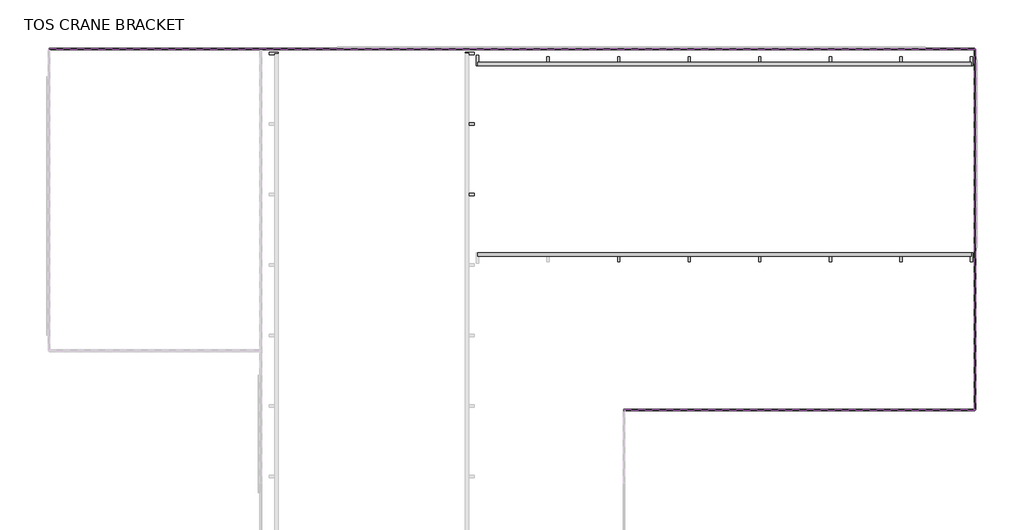
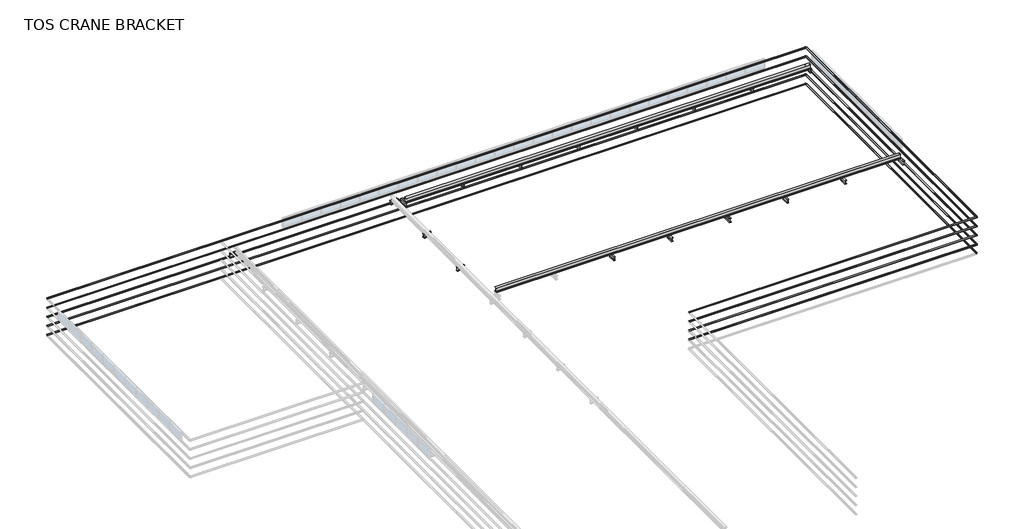
# One storey, part 3 of 3: 34 beams.
"""IFC4 building model written with IfcOpenShell, lengths in millimetres."""

import ifcopenshell
import ifcopenshell.guid

model = None  # the IFC model being written
_history = None  # IfcOwnerHistory: only IFC2X3 demands one
_inside = {}  # id of a spatial element -> (the spatial element, [elements in it])
_under = {}  # id of a project, library or spatial element -> (it, [spatial elements below it])
_declared = {}  # id of a project -> (the project, [libraries it declares])
_typed = {}  # id of a type object -> (the type object, [elements of that type])
_made_of = {}  # id of a material, layer set ... -> (it, [elements and type objects made of it])


def new_model(schema):
    """Start an empty IFC model of exactly this schema.

    Asked for "IFC4X3", IfcOpenShell would pick the latest addendum, in which some entities
    have other attributes; the version numbers below select the first issue.
    IFC2X3 requires an IfcOwnerHistory on every rooted entity: one is made here for all.
    """
    global model, _history
    if schema == "IFC4X3":
        model = ifcopenshell.file(schema_version=(4, 3, 0, 0))
    else:
        model = ifcopenshell.file(schema=schema)
    _inside.clear()
    _under.clear()
    _declared.clear()
    _typed.clear()
    _made_of.clear()
    _history = None
    if model.schema == "IFC2X3":
        org = make("IfcOrganization", Name="unknown")
        user = make(
            "IfcPersonAndOrganization",
            ThePerson=make("IfcPerson", FamilyName="unknown"),
            TheOrganization=org,
        )
        app = make(
            "IfcApplication",
            ApplicationDeveloper=org,
            Version="unknown",
            ApplicationFullName="unknown",
            ApplicationIdentifier="unknown",
        )
        _history = make(
            "IfcOwnerHistory",
            OwningUser=user,
            OwningApplication=app,
            ChangeAction="ADDED",
            CreationDate=0,
        )
    return model


def make(cls, **values):
    """One entity of the class cls with the attributes given. An attribute that is None is left unset."""
    return model.create_entity(
        cls, **{name: value for name, value in values.items() if value is not None}
    )


def rooted(cls, **values):
    """An entity with a GlobalId (a new one), such as an element, a storey or a relation."""
    return make(cls, GlobalId=ifcopenshell.guid.new(), OwnerHistory=_history, **values)


def si_unit(unit_type, name, prefix=None):
    """IfcSIUnit, for example si_unit("LENGTHUNIT", "METRE", prefix="MILLI")."""
    return make("IfcSIUnit", UnitType=unit_type, Prefix=prefix, Name=name)


def assignment(units):
    """IfcUnitAssignment: the units of a project."""
    return None if units is None else make("IfcUnitAssignment", Units=units)


def point(xyz):
    """IfcCartesianPoint."""
    return None if xyz is None else make("IfcCartesianPoint", Coordinates=xyz)


def direction(xyz):
    """IfcDirection."""
    return None if xyz is None else make("IfcDirection", DirectionRatios=xyz)


def frame(location, z_axis=None, x_axis=None):
    """IfcAxis2Placement3D, a coordinate frame: its origin and axes. An axis left out is left unset."""
    return make(
        "IfcAxis2Placement3D",
        Location=point(location),
        Axis=direction(z_axis),
        RefDirection=direction(x_axis),
    )


def frame_2d(location, x_axis=None):
    """IfcAxis2Placement2D, a coordinate frame in the plane: its origin and x axis."""
    return make(
        "IfcAxis2Placement2D", Location=point(location), RefDirection=direction(x_axis)
    )


def origin():
    """The frame at (0, 0, 0) with its axes left unset."""
    return frame((0.0, 0.0, 0.0))


def place(relative_to, where):
    """IfcLocalPlacement: puts the frame where relative to a parent placement (None: the world)."""
    return make(
        "IfcLocalPlacement", PlacementRelTo=relative_to, RelativePlacement=where
    )


def context(
    kind, dimensions, precision=None, world=None, true_north=None, identifier=None
):
    """IfcGeometricRepresentationContext, for example the 3D "Model" context."""
    return make(
        "IfcGeometricRepresentationContext",
        ContextIdentifier=identifier,
        ContextType=kind,
        CoordinateSpaceDimension=dimensions,
        Precision=precision,
        WorldCoordinateSystem=world,
        TrueNorth=true_north,
    )


def project(units=None, contexts=None):
    """IfcProject with its units and contexts."""
    return rooted(
        "IfcProject",
        Name="project",
        RepresentationContexts=contexts,
        UnitsInContext=assignment(units),
    )


def spatial(cls, under=None, at=None, **own):
    """A site, building, storey or space (cls), placed at a placement, below another one or the project."""
    s = rooted(cls, ObjectPlacement=at, **own)
    if under is not None:
        _under.setdefault(under.id(), (under, []))[1].append(s)
    return s


def polyline(points):
    """IfcPolyline through the points."""
    return make("IfcPolyline", Points=[point(p) for p in points])


def circle_curve(where, radius):
    """IfcCircle in the frame where."""
    return make("IfcCircle", Position=where, Radius=radius)


def trimmed(basis, trim1, trim2, sense, master):
    """IfcTrimmedCurve: the piece of a basis curve between two trims."""
    return make(
        "IfcTrimmedCurve",
        BasisCurve=basis,
        Trim1=trim1,
        Trim2=trim2,
        SenseAgreement=sense,
        MasterRepresentation=master,
    )


def segment(curve, same_sense, transition):
    """IfcCompositeCurveSegment."""
    return make(
        "IfcCompositeCurveSegment",
        Transition=transition,
        SameSense=same_sense,
        ParentCurve=curve,
    )


def composite_curve(segments, self_intersect=None):
    """IfcCompositeCurve: segments joined end to end."""
    return make("IfcCompositeCurve", Segments=segments, SelfIntersect=self_intersect)


def outline(outer, holes=None, kind="AREA"):
    """IfcArbitraryClosedProfileDef: a profile drawn as a closed curve; with holes, ...WithVoids."""
    if holes is None:
        return make("IfcArbitraryClosedProfileDef", ProfileType=kind, OuterCurve=outer)
    return make(
        "IfcArbitraryProfileDefWithVoids",
        ProfileType=kind,
        OuterCurve=outer,
        InnerCurves=holes,
    )


def extrude(swept, where, along, depth):
    """IfcExtrudedAreaSolid: the profile swept, set in the frame where, extruded along a direction by depth."""
    return make(
        "IfcExtrudedAreaSolid",
        SweptArea=swept,
        Position=where,
        ExtrudedDirection=direction(along),
        Depth=depth,
    )


def shape(context_of_items, identifier, shape_type, items):
    """IfcShapeRepresentation: the items that make up one representation, for example the "Body"."""
    return make(
        "IfcShapeRepresentation",
        ContextOfItems=context_of_items,
        RepresentationIdentifier=identifier,
        RepresentationType=shape_type,
        Items=items,
    )


def source(mapping_origin, context_of_items, identifier, shape_type, items):
    """IfcRepresentationMap: a shape defined once, which mapped items show again and again."""
    return make(
        "IfcRepresentationMap",
        MappingOrigin=mapping_origin,
        MappedRepresentation=shape(context_of_items, identifier, shape_type, items),
    )


def transform(
    local_origin,
    x_axis=None,
    y_axis=None,
    z_axis=None,
    scale=None,
    scale2=None,
    scale3=None,
    uniform=True,
):
    """IfcCartesianTransformationOperator3D, or its non-uniform kind. x_axis, y_axis, z_axis: its Axis1, 2, 3."""
    if uniform:
        return make(
            "IfcCartesianTransformationOperator3D",
            Axis1=direction(x_axis),
            Axis2=direction(y_axis),
            LocalOrigin=point(local_origin),
            Scale=scale,
            Axis3=direction(z_axis),
        )
    return make(
        "IfcCartesianTransformationOperator3DnonUniform",
        Axis1=direction(x_axis),
        Axis2=direction(y_axis),
        LocalOrigin=point(local_origin),
        Scale=scale,
        Axis3=direction(z_axis),
        Scale2=scale2,
        Scale3=scale3,
    )


def mapped(mapping_source, mapping_target):
    """IfcMappedItem: shows the shape of a source again, moved by a transform."""
    return make(
        "IfcMappedItem", MappingSource=mapping_source, MappingTarget=mapping_target
    )


def made_of(thing, what):
    """Note that an element or type object is made of a material, layer set ...; save() writes the relation."""
    if what is not None:
        _made_of.setdefault(what.id(), (what, []))[1].append(thing)
    return thing


def element(
    cls,
    number,
    at=None,
    inside=None,
    cuts=None,
    type_object=None,
    material=None,
    context=None,
    identifier="Body",
    shape_type=None,
    held_by="IfcProductDefinitionShape",
    body=None,
    shapes=None,
    **own,
):
    """One element of the class cls, such as IfcWall. Its Tag is "e" and its number.

    at: its placement. inside: the storey or other place that contains it. cuts: it is an
    opening in that element (IfcRelVoidsElement). A single representation is given by context,
    identifier, shape_type and body (its items); several are given by shapes. held_by: the class
    of the entity that holds the representations. save() writes the other relations.
    """
    e = rooted(cls, Tag="e%d" % number, ObjectPlacement=at, **own)
    if body is not None:
        shapes = [shape(context, identifier, shape_type, body)]
    if shapes is not None:
        e.Representation = make(held_by, Representations=shapes)
    if inside is not None:
        _inside.setdefault(inside.id(), (inside, []))[1].append(e)
    if cuts is not None:
        rooted(
            "IfcRelVoidsElement", RelatingBuildingElement=cuts, RelatedOpeningElement=e
        )
    if type_object is not None:
        _typed.setdefault(type_object.id(), (type_object, []))[1].append(e)
    return made_of(e, material)


def aggregate(whole, parts):
    """IfcRelAggregates: a whole, such as a stair, and the parts it consists of."""
    return rooted("IfcRelAggregates", RelatingObject=whole, RelatedObjects=parts)


def save(model, path):
    """Write the relations noted so far, then the file.

    IfcRelAggregates (storeys below a building ...), IfcRelContainedInSpatialStructure (elements
    in a storey), IfcRelDefinesByType, IfcRelAssociatesMaterial and IfcRelDeclares: one each for
    every whole, place, type object, material and project.
    """
    for whole, parts in _under.values():
        aggregate(whole, parts)
    for where, things in _inside.values():
        rooted(
            "IfcRelContainedInSpatialStructure",
            RelatedElements=things,
            RelatingStructure=where,
        )
    for kind, things in _typed.values():
        rooted("IfcRelDefinesByType", RelatedObjects=things, RelatingType=kind)
    for what, things in _made_of.values():
        rooted("IfcRelAssociatesMaterial", RelatedObjects=things, RelatingMaterial=what)
    for by, libraries in _declared.values():
        rooted("IfcRelDeclares", RelatingContext=by, RelatedDefinitions=libraries)
    model.write(path)


def beam_a081c7c9(model_context):
    return source(origin(), model_context, "Body", "SweptSolid", [
        extrude(outline(composite_curve([segment(polyline([(100.0, -187.0), (100.0, -200.0), (-100.0, -200.0), (-100.0, -187.0), (-20.0, -187.0)]), True, "CONTINUOUS"), segment(trimmed(circle_curve(frame_2d((-20.0, -171.0)), 16.0), [point((-20.0, -187.0))], [point((-4.0, -171.0))], True, "CARTESIAN"), True, "CONTINUOUS"), segment(polyline([(-4.0, -171.0), (-4.0, 171.0)]), True, "CONTINUOUS"), segment(trimmed(circle_curve(frame_2d((-20.0, 171.0)), 16.0), [point((-4.0, 171.0))], [point((-20.0, 187.0))], True, "CARTESIAN"), True, "CONTINUOUS"), segment(polyline([(-20.0, 187.0), (-100.0, 187.0), (-100.0, 200.0), (100.0, 200.0), (100.0, 187.0), (20.0, 187.0)]), True, "CONTINUOUS"), segment(trimmed(circle_curve(frame_2d((20.0, 171.0)), 16.0), [point((20.0, 187.0))], [point((4.0, 171.0))], True, "CARTESIAN"), True, "CONTINUOUS"), segment(polyline([(4.0, 171.0), (4.0, -171.0)]), True, "CONTINUOUS"), segment(trimmed(circle_curve(frame_2d((20.0, -171.0)), 16.0), [point((4.0, -171.0))], [point((20.0, -187.0))], True, "CARTESIAN"), True, "CONTINUOUS"), segment(polyline([(20.0, -187.0), (100.0, -187.0)]), True, "CONTINUOUS")], self_intersect=False)), frame((-236.0, 0.0, 0.0), z_axis=(1.0, 0.0, 0.0), x_axis=(0.0, 1.0, 0.0)), (0.0, 0.0, 1.0), 766.0),
    ])


def beam_d36fe593(model_context):
    return source(origin(), model_context, "Body", "SweptSolid", [
        extrude(outline(composite_curve([segment(polyline([(-100.0, -187.0), (-20.0, -187.0)]), True, "CONTINUOUS"), segment(trimmed(circle_curve(frame_2d((-20.0, -171.0)), 16.0), [point((-20.0, -187.0))], [point((-4.0, -171.0))], True, "CARTESIAN"), True, "CONTINUOUS"), segment(polyline([(-4.0, -171.0), (-4.0, 171.0)]), True, "CONTINUOUS"), segment(trimmed(circle_curve(frame_2d((-20.0, 171.0)), 16.0), [point((-4.0, 171.0))], [point((-20.0, 187.0))], True, "CARTESIAN"), True, "CONTINUOUS"), segment(polyline([(-20.0, 187.0), (-100.0, 187.0), (-100.0, 200.0), (100.0, 200.0), (100.0, 187.0), (20.0, 187.0)]), True, "CONTINUOUS"), segment(trimmed(circle_curve(frame_2d((20.0, 171.0)), 16.0), [point((20.0, 187.0))], [point((4.0, 171.0))], True, "CARTESIAN"), True, "CONTINUOUS"), segment(polyline([(4.0, 171.0), (4.0, -171.0)]), True, "CONTINUOUS"), segment(trimmed(circle_curve(frame_2d((20.0, -171.0)), 16.0), [point((4.0, -171.0))], [point((20.0, -187.0))], True, "CARTESIAN"), True, "CONTINUOUS"), segment(polyline([(20.0, -187.0), (100.0, -187.0), (100.0, -200.0), (-100.0, -200.0), (-100.0, -187.0)]), True, "CONTINUOUS")], self_intersect=False)), frame((-236.0, 0.0, 0.0), z_axis=(1.0, 0.0, 0.0), x_axis=(0.0, 1.0, 0.0)), (0.0, 0.0, 1.0), 766.0),
    ])


def beam_cf9155bb(model_context):
    return source(origin(), model_context, "Body", "SweptSolid", [
        extrude(outline(composite_curve([segment(polyline([(100.0, -187.0), (100.0, -200.0), (-100.0, -200.0), (-100.0, -187.0), (-20.0, -187.0)]), True, "CONTINUOUS"), segment(trimmed(circle_curve(frame_2d((-20.0, -171.0)), 16.0), [point((-20.0, -187.0))], [point((-4.0, -171.0))], True, "CARTESIAN"), True, "CONTINUOUS"), segment(polyline([(-4.0, -171.0), (-4.0, 171.0)]), True, "CONTINUOUS"), segment(trimmed(circle_curve(frame_2d((-20.0, 171.0)), 16.0), [point((-4.0, 171.0))], [point((-20.0, 187.0))], True, "CARTESIAN"), True, "CONTINUOUS"), segment(polyline([(-20.0, 187.0), (-100.0, 187.0), (-100.0, 200.0), (100.0, 200.0), (100.0, 187.0), (20.0, 187.0)]), True, "CONTINUOUS"), segment(trimmed(circle_curve(frame_2d((20.0, 171.0)), 16.0), [point((20.0, 187.0))], [point((4.0, 171.0))], True, "CARTESIAN"), True, "CONTINUOUS"), segment(polyline([(4.0, 171.0), (4.0, -171.0)]), True, "CONTINUOUS"), segment(trimmed(circle_curve(frame_2d((20.0, -171.0)), 16.0), [point((4.0, -171.0))], [point((20.0, -187.0))], True, "CARTESIAN"), True, "CONTINUOUS"), segment(polyline([(20.0, -187.0), (100.0, -187.0)]), True, "CONTINUOUS")], self_intersect=False)), frame((-380.0, 0.0, 0.0), z_axis=(1.0, 0.0, 0.0), x_axis=(0.0, 1.0, 0.0)), (0.0, 0.0, 1.0), 910.0),
    ])


def beam_632170ba(model_context):
    return source(origin(), model_context, "Body", "SweptSolid", [
        extrude(outline(composite_curve([segment(polyline([(150.0, -226.0), (150.0, -244.0), (-150.0, -244.0), (-150.0, -226.0), (-31.5, -226.0)]), True, "CONTINUOUS"), segment(trimmed(circle_curve(frame_2d((-31.5, -200.0)), 26.0), [point((-31.5, -226.0))], [point((-5.5, -200.0))], True, "CARTESIAN"), True, "CONTINUOUS"), segment(polyline([(-5.5, -200.0), (-5.5, 200.0)]), True, "CONTINUOUS"), segment(trimmed(circle_curve(frame_2d((-31.5, 200.0)), 26.0), [point((-5.5, 200.0))], [point((-31.5, 226.0))], True, "CARTESIAN"), True, "CONTINUOUS"), segment(polyline([(-31.5, 226.0), (-150.0, 226.0), (-150.0, 244.0), (150.0, 244.0), (150.0, 226.0), (31.5, 226.0)]), True, "CONTINUOUS"), segment(trimmed(circle_curve(frame_2d((31.5, 200.0)), 26.0), [point((31.5, 226.0))], [point((5.5, 200.0))], True, "CARTESIAN"), True, "CONTINUOUS"), segment(polyline([(5.5, 200.0), (5.5, -200.0)]), True, "CONTINUOUS"), segment(trimmed(circle_curve(frame_2d((31.5, -200.0)), 26.0), [point((5.5, -200.0))], [point((31.5, -226.0))], True, "CARTESIAN"), True, "CONTINUOUS"), segment(polyline([(31.5, -226.0), (150.0, -226.0)]), True, "CONTINUOUS")], self_intersect=False)), frame((-20987.2, 0.0, 0.0), z_axis=(1.0, 0.0, 0.0), x_axis=(0.0, 1.0, 0.0)), (0.0, 0.0, 1.0), 41974.4),
    ])


def beam_85a0d6c7(model_context):
    return source(origin(), model_context, "Body", "SweptSolid", [
        extrude(outline(composite_curve([segment(polyline([(-150.0, -226.0), (-31.5, -226.0)]), True, "CONTINUOUS"), segment(trimmed(circle_curve(frame_2d((-31.5, -200.0)), 26.0), [point((-31.5, -226.0))], [point((-5.5, -200.0))], True, "CARTESIAN"), True, "CONTINUOUS"), segment(polyline([(-5.5, -200.0), (-5.5, 200.0)]), True, "CONTINUOUS"), segment(trimmed(circle_curve(frame_2d((-31.5, 200.0)), 26.0), [point((-5.5, 200.0))], [point((-31.5, 226.0))], True, "CARTESIAN"), True, "CONTINUOUS"), segment(polyline([(-31.5, 226.0), (-150.0, 226.0), (-150.0, 244.0), (150.0, 244.0), (150.0, 226.0), (31.5, 226.0)]), True, "CONTINUOUS"), segment(trimmed(circle_curve(frame_2d((31.5, 200.0)), 26.0), [point((31.5, 226.0))], [point((5.5, 200.0))], True, "CARTESIAN"), True, "CONTINUOUS"), segment(polyline([(5.5, 200.0), (5.5, -200.0)]), True, "CONTINUOUS"), segment(trimmed(circle_curve(frame_2d((31.5, -200.0)), 26.0), [point((5.5, -200.0))], [point((31.5, -226.0))], True, "CARTESIAN"), True, "CONTINUOUS"), segment(polyline([(31.5, -226.0), (150.0, -226.0), (150.0, -244.0), (-150.0, -244.0), (-150.0, -226.0)]), True, "CONTINUOUS")], self_intersect=False)), frame((-20987.2, 0.0, 0.0), z_axis=(1.0, 0.0, 0.0), x_axis=(0.0, 1.0, 0.0)), (0.0, 0.0, 1.0), 41974.4),
    ])


def steel_framing_lc_01a803ec(model_context):
    return source(origin(), model_context, "Body", "SweptSolid", [
        extrude(outline(composite_curve([segment(polyline([(18.6, 67.0), (18.6, -67.0)]), True, "CONTINUOUS"), segment(trimmed(circle_curve(frame_2d((10.6, -67.0)), 8.0), [point((18.6, -67.0))], [point((10.6, -75.0))], False, "CARTESIAN"), True, "CONTINUOUS"), segment(polyline([(10.6, -75.0), (-48.4, -75.0)]), True, "CONTINUOUS"), segment(trimmed(circle_curve(frame_2d((-48.4, -67.0)), 8.0), [point((-48.4, -75.0))], [point((-56.4, -67.0))], False, "CARTESIAN"), True, "CONTINUOUS"), segment(polyline([(-56.4, -67.0), (-56.4, -50.0), (-53.2, -50.0), (-53.2, -67.0)]), True, "CONTINUOUS"), segment(trimmed(circle_curve(frame_2d((-48.4, -67.0)), 4.8), [point((-53.2, -67.0))], [point((-48.4, -71.8))], True, "CARTESIAN"), True, "CONTINUOUS"), segment(polyline([(-48.4, -71.8), (10.6, -71.8)]), True, "CONTINUOUS"), segment(trimmed(circle_curve(frame_2d((10.6, -67.0)), 4.8), [point((10.6, -71.8))], [point((15.4, -67.0))], True, "CARTESIAN"), True, "CONTINUOUS"), segment(polyline([(15.4, -67.0), (15.4, 67.0)]), True, "CONTINUOUS"), segment(trimmed(circle_curve(frame_2d((10.6, 67.0)), 4.8), [point((15.4, 67.0))], [point((10.6, 71.8))], True, "CARTESIAN"), True, "CONTINUOUS"), segment(polyline([(10.6, 71.8), (-48.4, 71.8)]), True, "CONTINUOUS"), segment(trimmed(circle_curve(frame_2d((-48.4, 67.0)), 4.8), [point((-48.4, 71.8))], [point((-53.2, 67.0))], True, "CARTESIAN"), True, "CONTINUOUS"), segment(polyline([(-53.2, 67.0), (-53.2, 50.0), (-56.4, 50.0), (-56.4, 67.0)]), True, "CONTINUOUS"), segment(trimmed(circle_curve(frame_2d((-48.4, 67.0)), 8.0), [point((-56.4, 67.0))], [point((-48.4, 75.0))], False, "CARTESIAN"), True, "CONTINUOUS"), segment(polyline([(-48.4, 75.0), (10.6, 75.0)]), True, "CONTINUOUS"), segment(trimmed(circle_curve(frame_2d((10.6, 67.0)), 8.0), [point((10.6, 75.0))], [point((18.6, 67.0))], False, "CARTESIAN"), True, "CONTINUOUS")], self_intersect=False)), frame((-39375.0, 0.0, 0.0), z_axis=(1.0, 0.0, 0.0), x_axis=(0.0, 1.0, 0.0)), (0.0, 0.0, 1.0), 78750.0),
    ])


model = new_model("IFC4")

# Units and contexts
model_context = context("Model", 3, world=origin())
ifc_project = project(units=[si_unit("LENGTHUNIT", "METRE", prefix="MILLI")], contexts=[model_context])

# Site, building, storey
site = spatial("IfcSite", under=ifc_project)
building = spatial("IfcBuilding", under=site)
storey = spatial("IfcBuildingStorey", under=building, Name="TOS CRANE BRACKET", Elevation=6699.9618634)

# Beams
placement = place(None, origin())
beam_shape = beam_a081c7c9(model_context)
element("IfcBeam", 1, ObjectType="Steel Framing_H_KS : H_SB_AR_S02_H-400x200x8x13_SCB1", at=placement, inside=storey, context=model_context, shape_type="MappedRepresentation", body=[
    mapped(beam_shape, transform((35470.0, -6000.0, 6499.9618634), x_axis=(-1.0, 0.0, 0.0), y_axis=(0.0, -1.0, 0.0), z_axis=(0.0, 0.0, 1.0))),
])
element("IfcBeam", 2, ObjectType="Steel Framing_H_KS : H_SB_AR_S02_H-400x200x8x13_SCB1", at=placement, inside=storey, context=model_context, shape_type="MappedRepresentation", body=[
    mapped(beam_shape, transform((35470.0, 0.0, 6499.9618634), x_axis=(-1.0, 0.0, 0.0), y_axis=(0.0, -1.0, 0.0), z_axis=(0.0, 0.0, 1.0))),
])
element("IfcBeam", 3, ObjectType="Steel Framing_H_KS : H_SB_AR_S02_H-400x200x8x13_SCB1", at=placement, inside=storey, context=model_context, shape_type="MappedRepresentation", body=[
    mapped(beam_shape, transform((35470.0, -12000.0, 6499.9618634), x_axis=(-1.0, 0.0, 0.0), y_axis=(0.0, -1.0, 0.0), z_axis=(0.0, 0.0, 1.0))),
])
element("IfcBeam", 4, ObjectType="Steel Framing_H_KS : H_SB_AR_S02_H-400x200x8x13_SCB1", at=placement, inside=storey, context=model_context, shape_type="MappedRepresentation", body=[
    mapped(beam_shape, transform((42000.0, -530.0, 6499.9618634), x_axis=(0.0, -1.0, 0.0), y_axis=(1.0, 0.0, 0.0), z_axis=(0.0, 0.0, 1.0))),
])
element("IfcBeam", 5, ObjectType="Steel Framing_H_KS : H_SB_AR_S02_H-400x200x8x13_SCB1", at=placement, inside=storey, context=model_context, shape_type="MappedRepresentation", body=[
    mapped(beam_shape, transform((48000.0, -530.0, 6499.9618634), x_axis=(0.0, -1.0, 0.0), y_axis=(1.0, 0.0, 0.0), z_axis=(0.0, 0.0, 1.0))),
])
element("IfcBeam", 6, ObjectType="Steel Framing_H_KS : H_SB_AR_S02_H-400x200x8x13_SCB1", at=placement, inside=storey, context=model_context, shape_type="MappedRepresentation", body=[
    mapped(beam_shape, transform((54000.0, -530.0, 6499.9618634), x_axis=(0.0, -1.0, 0.0), y_axis=(1.0, 0.0, 0.0), z_axis=(0.0, 0.0, 1.0))),
])
element("IfcBeam", 7, ObjectType="Steel Framing_H_KS : H_SB_AR_S02_H-400x200x8x13_SCB1", at=placement, inside=storey, context=model_context, shape_type="MappedRepresentation", body=[
    mapped(beam_shape, transform((60000.0, -530.0, 6499.9618634), x_axis=(0.0, -1.0, 0.0), y_axis=(1.0, 0.0, 0.0), z_axis=(0.0, 0.0, 1.0))),
])
element("IfcBeam", 8, ObjectType="Steel Framing_H_KS : H_SB_AR_S02_H-400x200x8x13_SCB1", at=placement, inside=storey, context=model_context, shape_type="MappedRepresentation", body=[
    mapped(beam_shape, transform((66000.0, -530.0, 6499.9618634), x_axis=(0.0, -1.0, 0.0), y_axis=(1.0, 0.0, 0.0), z_axis=(0.0, 0.0, 1.0))),
])
element("IfcBeam", 9, ObjectType="Steel Framing_H_KS : H_SB_AR_S02_H-400x200x8x13_SCB1", at=placement, inside=storey, context=model_context, shape_type="MappedRepresentation", body=[
    mapped(beam_shape, transform((72000.0, -530.0, 6499.9618634), x_axis=(0.0, -1.0, 0.0), y_axis=(1.0, 0.0, 0.0), z_axis=(0.0, 0.0, 1.0))),
])
element("IfcBeam", 10, ObjectType="Steel Framing_H_KS : H_SB_AR_S02_H-400x200x8x13_SCB1", at=placement, inside=storey, context=model_context, shape_type="MappedRepresentation", body=[
    mapped(beam_shape, transform((78000.0, -530.0, 6499.9618634), x_axis=(0.0, -1.0, 0.0), y_axis=(1.0, 0.0, 0.0), z_axis=(0.0, 0.0, 1.0))),
])
beam_2_shape = beam_d36fe593(model_context)
element("IfcBeam", 11, ObjectType="Steel Framing_H_KS : H_SB_AR_S02_H-400x200x8x13_SCB1", at=placement, inside=storey, context=model_context, shape_type="MappedRepresentation", body=[
    mapped(beam_2_shape, transform((18530.0, 0.0, 6499.9618634), x_axis=(1.0, 0.0, 0.0), y_axis=(0.0, 1.0, 0.0), z_axis=(0.0, 0.0, 1.0))),
])
element("IfcBeam", 12, ObjectType="Steel Framing_H_KS : H_SB_AR_S02_H-400x200x8x13_SCB1", at=placement, inside=storey, context=model_context, shape_type="MappedRepresentation", body=[
    mapped(beam_2_shape, transform((48000.0, -17470.0, 6499.9618634), x_axis=(0.0, 1.0, 0.0), y_axis=(-1.0, 0.0, 0.0), z_axis=(0.0, 0.0, 1.0))),
])
element("IfcBeam", 13, ObjectType="Steel Framing_H_KS : H_SB_AR_S02_H-400x200x8x13_SCB1", at=placement, inside=storey, context=model_context, shape_type="MappedRepresentation", body=[
    mapped(beam_2_shape, transform((54000.0, -17470.0, 6499.9618634), x_axis=(0.0, 1.0, 0.0), y_axis=(-1.0, 0.0, 0.0), z_axis=(0.0, 0.0, 1.0))),
])
element("IfcBeam", 14, ObjectType="Steel Framing_H_KS : H_SB_AR_S02_H-400x200x8x13_SCB1", at=placement, inside=storey, context=model_context, shape_type="MappedRepresentation", body=[
    mapped(beam_2_shape, transform((60000.0, -17470.0, 6499.9618634), x_axis=(0.0, 1.0, 0.0), y_axis=(-1.0, 0.0, 0.0), z_axis=(0.0, 0.0, 1.0))),
])
element("IfcBeam", 15, ObjectType="Steel Framing_H_KS : H_SB_AR_S02_H-400x200x8x13_SCB1", at=placement, inside=storey, context=model_context, shape_type="MappedRepresentation", body=[
    mapped(beam_2_shape, transform((66000.0, -17470.0, 6499.9618634), x_axis=(0.0, 1.0, 0.0), y_axis=(-1.0, 0.0, 0.0), z_axis=(0.0, 0.0, 1.0))),
])
element("IfcBeam", 16, ObjectType="Steel Framing_H_KS : H_SB_AR_S02_H-400x200x8x13_SCB1", at=placement, inside=storey, context=model_context, shape_type="MappedRepresentation", body=[
    mapped(beam_2_shape, transform((72000.0, -17470.0, 6499.9618634), x_axis=(0.0, 1.0, 0.0), y_axis=(-1.0, 0.0, 0.0), z_axis=(0.0, 0.0, 1.0))),
])
element("IfcBeam", 17, ObjectType="Steel Framing_H_KS : H_SB_AR_S02_H-400x200x8x13_SCB1", at=placement, inside=storey, context=model_context, shape_type="MappedRepresentation", body=[
    mapped(beam_2_shape, transform((78000.0, -17470.0, 6499.9618634), x_axis=(0.0, 1.0, 0.0), y_axis=(-1.0, 0.0, 0.0), z_axis=(0.0, 0.0, 1.0))),
])
beam_3_shape = beam_cf9155bb(model_context)
element("IfcBeam", 18, ObjectType="Steel Framing_H_KS : H_SB_AR_S02_H-400x200x8x13_SCB1", at=placement, inside=storey, context=model_context, shape_type="MappedRepresentation", body=[
    mapped(beam_3_shape, transform((36000.0, -530.0, 6499.9618634), x_axis=(0.0, -1.0, 0.0), y_axis=(1.0, 0.0, 0.0), z_axis=(0.0, 0.0, 1.0))),
])
beam_4_shape = beam_632170ba(model_context)
element("IfcBeam", 19, ObjectType="Steel Framing_H_KS : H_SB_AR_S02_H-488x300x11x18_CRG1", at=placement, inside=storey, context=model_context, shape_type="MappedRepresentation", body=[
    mapped(beam_4_shape, transform((57000.0, -900.0, 6953.9618634), x_axis=(1.0, 0.0, 0.0), y_axis=(0.0, 1.0, 0.0), z_axis=(0.0, 0.0, 1.0))),
])
beam_5_shape = beam_85a0d6c7(model_context)
element("IfcBeam", 20, ObjectType="Steel Framing_H_KS : H_SB_AR_S02_H-488x300x11x18_CRG1", at=placement, inside=storey, context=model_context, shape_type="MappedRepresentation", body=[
    mapped(beam_5_shape, transform((57000.0, -17100.0, 6953.9618634), x_axis=(1.0, 0.0, 0.0), y_axis=(0.0, 1.0, 0.0), z_axis=(0.0, 0.0, 1.0))),
])
element("IfcBeam", 21, ObjectType="Steel Framing_LC : H_SB_AR_S00_LC-150x75x25x3.2", at=placement, inside=storey, context=model_context, shape_type="SweptSolid", body=[
    extrude(outline(composite_curve([segment(trimmed(circle_curve(frame_2d((4160.5618634, 78233.0)), 8.0), [point((4168.5618634, 78233.0))], [point((4160.5618634, 78225.0))], False, "CARTESIAN"), True, "CONTINUOUS"), segment(polyline([(4160.5618634, 78225.0), (4101.5618634, 78225.0)]), True, "CONTINUOUS"), segment(trimmed(circle_curve(frame_2d((4101.5618634, 78233.0)), 8.0), [point((4101.5618634, 78225.0))], [point((4093.5618634, 78233.0))], False, "CARTESIAN"), True, "CONTINUOUS"), segment(polyline([(4093.5618634, 78233.0), (4093.5618634, 78250.0), (4096.7618634, 78250.0), (4096.7618634, 78233.0)]), True, "CONTINUOUS"), segment(trimmed(circle_curve(frame_2d((4101.5618634, 78233.0)), 4.8), [point((4096.7618634, 78233.0))], [point((4101.5618634, 78228.2))], True, "CARTESIAN"), True, "CONTINUOUS"), segment(polyline([(4101.5618634, 78228.2), (4160.5618634, 78228.2)]), True, "CONTINUOUS"), segment(trimmed(circle_curve(frame_2d((4160.5618634, 78233.0)), 4.8), [point((4160.5618634, 78228.2))], [point((4165.3618634, 78233.0))], True, "CARTESIAN"), True, "CONTINUOUS"), segment(polyline([(4165.3618634, 78233.0), (4165.3618634, 78367.0)]), True, "CONTINUOUS"), segment(trimmed(circle_curve(frame_2d((4160.5618634, 78367.0)), 4.8), [point((4165.3618634, 78367.0))], [point((4160.5618634, 78371.8))], True, "CARTESIAN"), True, "CONTINUOUS"), segment(polyline([(4160.5618634, 78371.8), (4101.5618634, 78371.8)]), True, "CONTINUOUS"), segment(trimmed(circle_curve(frame_2d((4101.5618634, 78367.0)), 4.8), [point((4101.5618634, 78371.8))], [point((4096.7618634, 78367.0))], True, "CARTESIAN"), True, "CONTINUOUS"), segment(polyline([(4096.7618634, 78367.0), (4096.7618634, 78350.0), (4093.5618634, 78350.0), (4093.5618634, 78367.0)]), True, "CONTINUOUS"), segment(trimmed(circle_curve(frame_2d((4101.5618634, 78367.0)), 8.0), [point((4093.5618634, 78367.0))], [point((4101.5618634, 78375.0))], False, "CARTESIAN"), True, "CONTINUOUS"), segment(polyline([(4101.5618634, 78375.0), (4160.5618634, 78375.0)]), True, "CONTINUOUS"), segment(trimmed(circle_curve(frame_2d((4160.5618634, 78367.0)), 8.0), [point((4160.5618634, 78375.0))], [point((4168.5618634, 78367.0))], False, "CARTESIAN"), True, "CONTINUOUS"), segment(polyline([(4168.5618634, 78367.0), (4168.5618634, 78233.0)]), True, "CONTINUOUS")], self_intersect=False)), frame((0.0, -30325.0, 0.0), z_axis=(0.0, 1.0, 0.0), x_axis=(0.0, 0.0, 1.0)), (0.0, 0.0, 1.0), 30694.0),
])
element("IfcBeam", 22, ObjectType="Steel Framing_LC : H_SB_AR_S00_LC-150x75x25x3.2", at=placement, inside=storey, context=model_context, shape_type="SweptSolid", body=[
    extrude(outline(composite_curve([segment(trimmed(circle_curve(frame_2d((5160.5618634, 78233.0)), 8.0), [point((5168.5618634, 78233.0))], [point((5160.5618634, 78225.0))], False, "CARTESIAN"), True, "CONTINUOUS"), segment(polyline([(5160.5618634, 78225.0), (5101.5618634, 78225.0)]), True, "CONTINUOUS"), segment(trimmed(circle_curve(frame_2d((5101.5618634, 78233.0)), 8.0), [point((5101.5618634, 78225.0))], [point((5093.5618634, 78233.0))], False, "CARTESIAN"), True, "CONTINUOUS"), segment(polyline([(5093.5618634, 78233.0), (5093.5618634, 78250.0), (5096.7618634, 78250.0), (5096.7618634, 78233.0)]), True, "CONTINUOUS"), segment(trimmed(circle_curve(frame_2d((5101.5618634, 78233.0)), 4.8), [point((5096.7618634, 78233.0))], [point((5101.5618634, 78228.2))], True, "CARTESIAN"), True, "CONTINUOUS"), segment(polyline([(5101.5618634, 78228.2), (5160.5618634, 78228.2)]), True, "CONTINUOUS"), segment(trimmed(circle_curve(frame_2d((5160.5618634, 78233.0)), 4.8), [point((5160.5618634, 78228.2))], [point((5165.3618634, 78233.0))], True, "CARTESIAN"), True, "CONTINUOUS"), segment(polyline([(5165.3618634, 78233.0), (5165.3618634, 78367.0)]), True, "CONTINUOUS"), segment(trimmed(circle_curve(frame_2d((5160.5618634, 78367.0)), 4.8), [point((5165.3618634, 78367.0))], [point((5160.5618634, 78371.8))], True, "CARTESIAN"), True, "CONTINUOUS"), segment(polyline([(5160.5618634, 78371.8), (5101.5618634, 78371.8)]), True, "CONTINUOUS"), segment(trimmed(circle_curve(frame_2d((5101.5618634, 78367.0)), 4.8), [point((5101.5618634, 78371.8))], [point((5096.7618634, 78367.0))], True, "CARTESIAN"), True, "CONTINUOUS"), segment(polyline([(5096.7618634, 78367.0), (5096.7618634, 78350.0), (5093.5618634, 78350.0), (5093.5618634, 78367.0)]), True, "CONTINUOUS"), segment(trimmed(circle_curve(frame_2d((5101.5618634, 78367.0)), 8.0), [point((5093.5618634, 78367.0))], [point((5101.5618634, 78375.0))], False, "CARTESIAN"), True, "CONTINUOUS"), segment(polyline([(5101.5618634, 78375.0), (5160.5618634, 78375.0)]), True, "CONTINUOUS"), segment(trimmed(circle_curve(frame_2d((5160.5618634, 78367.0)), 8.0), [point((5160.5618634, 78375.0))], [point((5168.5618634, 78367.0))], False, "CARTESIAN"), True, "CONTINUOUS"), segment(polyline([(5168.5618634, 78367.0), (5168.5618634, 78233.0)]), True, "CONTINUOUS")], self_intersect=False)), frame((0.0, -30325.0, 0.0), z_axis=(0.0, 1.0, 0.0), x_axis=(0.0, 0.0, 1.0)), (0.0, 0.0, 1.0), 30694.0),
])
element("IfcBeam", 23, ObjectType="Steel Framing_LC : H_SB_AR_S00_LC-150x75x25x3.2", at=placement, inside=storey, context=model_context, shape_type="SweptSolid", body=[
    extrude(outline(composite_curve([segment(polyline([(-30392.0, 5168.5618634), (-30258.0, 5168.5618634)]), True, "CONTINUOUS"), segment(trimmed(circle_curve(frame_2d((-30258.0, 5160.5618634)), 8.0), [point((-30258.0, 5168.5618634))], [point((-30250.0, 5160.5618634))], False, "CARTESIAN"), True, "CONTINUOUS"), segment(polyline([(-30250.0, 5160.5618634), (-30250.0, 5101.5618634)]), True, "CONTINUOUS"), segment(trimmed(circle_curve(frame_2d((-30258.0, 5101.5618634)), 8.0), [point((-30250.0, 5101.5618634))], [point((-30258.0, 5093.5618634))], False, "CARTESIAN"), True, "CONTINUOUS"), segment(polyline([(-30258.0, 5093.5618634), (-30275.0, 5093.5618634), (-30275.0, 5096.7618634), (-30258.0, 5096.7618634)]), True, "CONTINUOUS"), segment(trimmed(circle_curve(frame_2d((-30258.0, 5101.5618634)), 4.8), [point((-30258.0, 5096.7618634))], [point((-30253.2, 5101.5618634))], True, "CARTESIAN"), True, "CONTINUOUS"), segment(polyline([(-30253.2, 5101.5618634), (-30253.2, 5160.5618634)]), True, "CONTINUOUS"), segment(trimmed(circle_curve(frame_2d((-30258.0, 5160.5618634)), 4.8), [point((-30253.2, 5160.5618634))], [point((-30258.0, 5165.3618634))], True, "CARTESIAN"), True, "CONTINUOUS"), segment(polyline([(-30258.0, 5165.3618634), (-30392.0, 5165.3618634)]), True, "CONTINUOUS"), segment(trimmed(circle_curve(frame_2d((-30392.0, 5160.5618634)), 4.8), [point((-30392.0, 5165.3618634))], [point((-30396.8, 5160.5618634))], True, "CARTESIAN"), True, "CONTINUOUS"), segment(polyline([(-30396.8, 5160.5618634), (-30396.8, 5101.5618634)]), True, "CONTINUOUS"), segment(trimmed(circle_curve(frame_2d((-30392.0, 5101.5618634)), 4.8), [point((-30396.8, 5101.5618634))], [point((-30392.0, 5096.7618634))], True, "CARTESIAN"), True, "CONTINUOUS"), segment(polyline([(-30392.0, 5096.7618634), (-30375.0, 5096.7618634), (-30375.0, 5093.5618634), (-30392.0, 5093.5618634)]), True, "CONTINUOUS"), segment(trimmed(circle_curve(frame_2d((-30392.0, 5101.5618634)), 8.0), [point((-30392.0, 5093.5618634))], [point((-30400.0, 5101.5618634))], False, "CARTESIAN"), True, "CONTINUOUS"), segment(polyline([(-30400.0, 5101.5618634), (-30400.0, 5160.5618634)]), True, "CONTINUOUS"), segment(trimmed(circle_curve(frame_2d((-30392.0, 5160.5618634)), 8.0), [point((-30400.0, 5160.5618634))], [point((-30392.0, 5168.5618634))], False, "CARTESIAN"), True, "CONTINUOUS")], self_intersect=False)), frame((48450.0, 0.0, 0.0), z_axis=(1.0, 0.0, 0.0), x_axis=(0.0, 1.0, 0.0)), (0.0, 0.0, 1.0), 29850.0),
])
element("IfcBeam", 24, ObjectType="Steel Framing_LC : H_SB_AR_S00_LC-150x75x25x3.2", at=placement, inside=storey, context=model_context, shape_type="SweptSolid", body=[
    extrude(outline(composite_curve([segment(trimmed(circle_curve(frame_2d((6160.5618634, 78233.0)), 8.0), [point((6168.5618634, 78233.0))], [point((6160.5618634, 78225.0))], False, "CARTESIAN"), True, "CONTINUOUS"), segment(polyline([(6160.5618634, 78225.0), (6101.5618634, 78225.0)]), True, "CONTINUOUS"), segment(trimmed(circle_curve(frame_2d((6101.5618634, 78233.0)), 8.0), [point((6101.5618634, 78225.0))], [point((6093.5618634, 78233.0))], False, "CARTESIAN"), True, "CONTINUOUS"), segment(polyline([(6093.5618634, 78233.0), (6093.5618634, 78250.0), (6096.7618634, 78250.0), (6096.7618634, 78233.0)]), True, "CONTINUOUS"), segment(trimmed(circle_curve(frame_2d((6101.5618634, 78233.0)), 4.8), [point((6096.7618634, 78233.0))], [point((6101.5618634, 78228.2))], True, "CARTESIAN"), True, "CONTINUOUS"), segment(polyline([(6101.5618634, 78228.2), (6160.5618634, 78228.2)]), True, "CONTINUOUS"), segment(trimmed(circle_curve(frame_2d((6160.5618634, 78233.0)), 4.8), [point((6160.5618634, 78228.2))], [point((6165.3618634, 78233.0))], True, "CARTESIAN"), True, "CONTINUOUS"), segment(polyline([(6165.3618634, 78233.0), (6165.3618634, 78367.0)]), True, "CONTINUOUS"), segment(trimmed(circle_curve(frame_2d((6160.5618634, 78367.0)), 4.8), [point((6165.3618634, 78367.0))], [point((6160.5618634, 78371.8))], True, "CARTESIAN"), True, "CONTINUOUS"), segment(polyline([(6160.5618634, 78371.8), (6101.5618634, 78371.8)]), True, "CONTINUOUS"), segment(trimmed(circle_curve(frame_2d((6101.5618634, 78367.0)), 4.8), [point((6101.5618634, 78371.8))], [point((6096.7618634, 78367.0))], True, "CARTESIAN"), True, "CONTINUOUS"), segment(polyline([(6096.7618634, 78367.0), (6096.7618634, 78350.0), (6093.5618634, 78350.0), (6093.5618634, 78367.0)]), True, "CONTINUOUS"), segment(trimmed(circle_curve(frame_2d((6101.5618634, 78367.0)), 8.0), [point((6093.5618634, 78367.0))], [point((6101.5618634, 78375.0))], False, "CARTESIAN"), True, "CONTINUOUS"), segment(polyline([(6101.5618634, 78375.0), (6160.5618634, 78375.0)]), True, "CONTINUOUS"), segment(trimmed(circle_curve(frame_2d((6160.5618634, 78367.0)), 8.0), [point((6160.5618634, 78375.0))], [point((6168.5618634, 78367.0))], False, "CARTESIAN"), True, "CONTINUOUS"), segment(polyline([(6168.5618634, 78367.0), (6168.5618634, 78233.0)]), True, "CONTINUOUS")], self_intersect=False)), frame((0.0, -30325.0, 0.0), z_axis=(0.0, 1.0, 0.0), x_axis=(0.0, 0.0, 1.0)), (0.0, 0.0, 1.0), 30694.0),
])
element("IfcBeam", 25, ObjectType="Steel Framing_LC : H_SB_AR_S00_LC-150x75x25x3.2", at=placement, inside=storey, context=model_context, shape_type="SweptSolid", body=[
    extrude(outline(composite_curve([segment(polyline([(-30392.0, 6168.5618634), (-30258.0, 6168.5618634)]), True, "CONTINUOUS"), segment(trimmed(circle_curve(frame_2d((-30258.0, 6160.5618634)), 8.0), [point((-30258.0, 6168.5618634))], [point((-30250.0, 6160.5618634))], False, "CARTESIAN"), True, "CONTINUOUS"), segment(polyline([(-30250.0, 6160.5618634), (-30250.0, 6101.5618634)]), True, "CONTINUOUS"), segment(trimmed(circle_curve(frame_2d((-30258.0, 6101.5618634)), 8.0), [point((-30250.0, 6101.5618634))], [point((-30258.0, 6093.5618634))], False, "CARTESIAN"), True, "CONTINUOUS"), segment(polyline([(-30258.0, 6093.5618634), (-30275.0, 6093.5618634), (-30275.0, 6096.7618634), (-30258.0, 6096.7618634)]), True, "CONTINUOUS"), segment(trimmed(circle_curve(frame_2d((-30258.0, 6101.5618634)), 4.8), [point((-30258.0, 6096.7618634))], [point((-30253.2, 6101.5618634))], True, "CARTESIAN"), True, "CONTINUOUS"), segment(polyline([(-30253.2, 6101.5618634), (-30253.2, 6160.5618634)]), True, "CONTINUOUS"), segment(trimmed(circle_curve(frame_2d((-30258.0, 6160.5618634)), 4.8), [point((-30253.2, 6160.5618634))], [point((-30258.0, 6165.3618634))], True, "CARTESIAN"), True, "CONTINUOUS"), segment(polyline([(-30258.0, 6165.3618634), (-30392.0, 6165.3618634)]), True, "CONTINUOUS"), segment(trimmed(circle_curve(frame_2d((-30392.0, 6160.5618634)), 4.8), [point((-30392.0, 6165.3618634))], [point((-30396.8, 6160.5618634))], True, "CARTESIAN"), True, "CONTINUOUS"), segment(polyline([(-30396.8, 6160.5618634), (-30396.8, 6101.5618634)]), True, "CONTINUOUS"), segment(trimmed(circle_curve(frame_2d((-30392.0, 6101.5618634)), 4.8), [point((-30396.8, 6101.5618634))], [point((-30392.0, 6096.7618634))], True, "CARTESIAN"), True, "CONTINUOUS"), segment(polyline([(-30392.0, 6096.7618634), (-30375.0, 6096.7618634), (-30375.0, 6093.5618634), (-30392.0, 6093.5618634)]), True, "CONTINUOUS"), segment(trimmed(circle_curve(frame_2d((-30392.0, 6101.5618634)), 8.0), [point((-30392.0, 6093.5618634))], [point((-30400.0, 6101.5618634))], False, "CARTESIAN"), True, "CONTINUOUS"), segment(polyline([(-30400.0, 6101.5618634), (-30400.0, 6160.5618634)]), True, "CONTINUOUS"), segment(trimmed(circle_curve(frame_2d((-30392.0, 6160.5618634)), 8.0), [point((-30400.0, 6160.5618634))], [point((-30392.0, 6168.5618634))], False, "CARTESIAN"), True, "CONTINUOUS")], self_intersect=False)), frame((48450.0, 0.0, 0.0), z_axis=(1.0, 0.0, 0.0), x_axis=(0.0, 1.0, 0.0)), (0.0, 0.0, 1.0), 29850.0),
])
element("IfcBeam", 26, ObjectType="Steel Framing_LC : H_SB_AR_S00_LC-150x75x25x3.2", at=placement, inside=storey, context=model_context, shape_type="SweptSolid", body=[
    extrude(outline(composite_curve([segment(trimmed(circle_curve(frame_2d((7160.5618634, 78233.0)), 8.0), [point((7168.5618634, 78233.0))], [point((7160.5618634, 78225.0))], False, "CARTESIAN"), True, "CONTINUOUS"), segment(polyline([(7160.5618634, 78225.0), (7101.5618634, 78225.0)]), True, "CONTINUOUS"), segment(trimmed(circle_curve(frame_2d((7101.5618634, 78233.0)), 8.0), [point((7101.5618634, 78225.0))], [point((7093.5618634, 78233.0))], False, "CARTESIAN"), True, "CONTINUOUS"), segment(polyline([(7093.5618634, 78233.0), (7093.5618634, 78250.0), (7096.7618634, 78250.0), (7096.7618634, 78233.0)]), True, "CONTINUOUS"), segment(trimmed(circle_curve(frame_2d((7101.5618634, 78233.0)), 4.8), [point((7096.7618634, 78233.0))], [point((7101.5618634, 78228.2))], True, "CARTESIAN"), True, "CONTINUOUS"), segment(polyline([(7101.5618634, 78228.2), (7160.5618634, 78228.2)]), True, "CONTINUOUS"), segment(trimmed(circle_curve(frame_2d((7160.5618634, 78233.0)), 4.8), [point((7160.5618634, 78228.2))], [point((7165.3618634, 78233.0))], True, "CARTESIAN"), True, "CONTINUOUS"), segment(polyline([(7165.3618634, 78233.0), (7165.3618634, 78367.0)]), True, "CONTINUOUS"), segment(trimmed(circle_curve(frame_2d((7160.5618634, 78367.0)), 4.8), [point((7165.3618634, 78367.0))], [point((7160.5618634, 78371.8))], True, "CARTESIAN"), True, "CONTINUOUS"), segment(polyline([(7160.5618634, 78371.8), (7101.5618634, 78371.8)]), True, "CONTINUOUS"), segment(trimmed(circle_curve(frame_2d((7101.5618634, 78367.0)), 4.8), [point((7101.5618634, 78371.8))], [point((7096.7618634, 78367.0))], True, "CARTESIAN"), True, "CONTINUOUS"), segment(polyline([(7096.7618634, 78367.0), (7096.7618634, 78350.0), (7093.5618634, 78350.0), (7093.5618634, 78367.0)]), True, "CONTINUOUS"), segment(trimmed(circle_curve(frame_2d((7101.5618634, 78367.0)), 8.0), [point((7093.5618634, 78367.0))], [point((7101.5618634, 78375.0))], False, "CARTESIAN"), True, "CONTINUOUS"), segment(polyline([(7101.5618634, 78375.0), (7160.5618634, 78375.0)]), True, "CONTINUOUS"), segment(trimmed(circle_curve(frame_2d((7160.5618634, 78367.0)), 8.0), [point((7160.5618634, 78375.0))], [point((7168.5618634, 78367.0))], False, "CARTESIAN"), True, "CONTINUOUS"), segment(polyline([(7168.5618634, 78367.0), (7168.5618634, 78233.0)]), True, "CONTINUOUS")], self_intersect=False)), frame((0.0, -30325.0, 0.0), z_axis=(0.0, 1.0, 0.0), x_axis=(0.0, 0.0, 1.0)), (0.0, 0.0, 1.0), 30694.0),
])
element("IfcBeam", 27, ObjectType="Steel Framing_LC : H_SB_AR_S00_LC-150x75x25x3.2", at=placement, inside=storey, context=model_context, shape_type="SweptSolid", body=[
    extrude(outline(composite_curve([segment(polyline([(-30392.0, 7168.5618634), (-30258.0, 7168.5618634)]), True, "CONTINUOUS"), segment(trimmed(circle_curve(frame_2d((-30258.0, 7160.5618634)), 8.0), [point((-30258.0, 7168.5618634))], [point((-30250.0, 7160.5618634))], False, "CARTESIAN"), True, "CONTINUOUS"), segment(polyline([(-30250.0, 7160.5618634), (-30250.0, 7101.5618634)]), True, "CONTINUOUS"), segment(trimmed(circle_curve(frame_2d((-30258.0, 7101.5618634)), 8.0), [point((-30250.0, 7101.5618634))], [point((-30258.0, 7093.5618634))], False, "CARTESIAN"), True, "CONTINUOUS"), segment(polyline([(-30258.0, 7093.5618634), (-30275.0, 7093.5618634), (-30275.0, 7096.7618634), (-30258.0, 7096.7618634)]), True, "CONTINUOUS"), segment(trimmed(circle_curve(frame_2d((-30258.0, 7101.5618634)), 4.8), [point((-30258.0, 7096.7618634))], [point((-30253.2, 7101.5618634))], True, "CARTESIAN"), True, "CONTINUOUS"), segment(polyline([(-30253.2, 7101.5618634), (-30253.2, 7160.5618634)]), True, "CONTINUOUS"), segment(trimmed(circle_curve(frame_2d((-30258.0, 7160.5618634)), 4.8), [point((-30253.2, 7160.5618634))], [point((-30258.0, 7165.3618634))], True, "CARTESIAN"), True, "CONTINUOUS"), segment(polyline([(-30258.0, 7165.3618634), (-30392.0, 7165.3618634)]), True, "CONTINUOUS"), segment(trimmed(circle_curve(frame_2d((-30392.0, 7160.5618634)), 4.8), [point((-30392.0, 7165.3618634))], [point((-30396.8, 7160.5618634))], True, "CARTESIAN"), True, "CONTINUOUS"), segment(polyline([(-30396.8, 7160.5618634), (-30396.8, 7101.5618634)]), True, "CONTINUOUS"), segment(trimmed(circle_curve(frame_2d((-30392.0, 7101.5618634)), 4.8), [point((-30396.8, 7101.5618634))], [point((-30392.0, 7096.7618634))], True, "CARTESIAN"), True, "CONTINUOUS"), segment(polyline([(-30392.0, 7096.7618634), (-30375.0, 7096.7618634), (-30375.0, 7093.5618634), (-30392.0, 7093.5618634)]), True, "CONTINUOUS"), segment(trimmed(circle_curve(frame_2d((-30392.0, 7101.5618634)), 8.0), [point((-30392.0, 7093.5618634))], [point((-30400.0, 7101.5618634))], False, "CARTESIAN"), True, "CONTINUOUS"), segment(polyline([(-30400.0, 7101.5618634), (-30400.0, 7160.5618634)]), True, "CONTINUOUS"), segment(trimmed(circle_curve(frame_2d((-30392.0, 7160.5618634)), 8.0), [point((-30400.0, 7160.5618634))], [point((-30392.0, 7168.5618634))], False, "CARTESIAN"), True, "CONTINUOUS")], self_intersect=False)), frame((48450.0, 0.0, 0.0), z_axis=(1.0, 0.0, 0.0), x_axis=(0.0, 1.0, 0.0)), (0.0, 0.0, 1.0), 29850.0),
])
element("IfcBeam", 28, ObjectType="Steel Framing_LC : H_SB_AR_S00_LC-150x75x25x3.2", at=placement, inside=storey, context=model_context, shape_type="SweptSolid", body=[
    extrude(outline(composite_curve([segment(trimmed(circle_curve(frame_2d((8160.5618634, 78233.0)), 8.0), [point((8168.5618634, 78233.0))], [point((8160.5618634, 78225.0))], False, "CARTESIAN"), True, "CONTINUOUS"), segment(polyline([(8160.5618634, 78225.0), (8101.5618634, 78225.0)]), True, "CONTINUOUS"), segment(trimmed(circle_curve(frame_2d((8101.5618634, 78233.0)), 8.0), [point((8101.5618634, 78225.0))], [point((8093.5618634, 78233.0))], False, "CARTESIAN"), True, "CONTINUOUS"), segment(polyline([(8093.5618634, 78233.0), (8093.5618634, 78250.0), (8096.7618634, 78250.0), (8096.7618634, 78233.0)]), True, "CONTINUOUS"), segment(trimmed(circle_curve(frame_2d((8101.5618634, 78233.0)), 4.8), [point((8096.7618634, 78233.0))], [point((8101.5618634, 78228.2))], True, "CARTESIAN"), True, "CONTINUOUS"), segment(polyline([(8101.5618634, 78228.2), (8160.5618634, 78228.2)]), True, "CONTINUOUS"), segment(trimmed(circle_curve(frame_2d((8160.5618634, 78233.0)), 4.8), [point((8160.5618634, 78228.2))], [point((8165.3618634, 78233.0))], True, "CARTESIAN"), True, "CONTINUOUS"), segment(polyline([(8165.3618634, 78233.0), (8165.3618634, 78367.0)]), True, "CONTINUOUS"), segment(trimmed(circle_curve(frame_2d((8160.5618634, 78367.0)), 4.8), [point((8165.3618634, 78367.0))], [point((8160.5618634, 78371.8))], True, "CARTESIAN"), True, "CONTINUOUS"), segment(polyline([(8160.5618634, 78371.8), (8101.5618634, 78371.8)]), True, "CONTINUOUS"), segment(trimmed(circle_curve(frame_2d((8101.5618634, 78367.0)), 4.8), [point((8101.5618634, 78371.8))], [point((8096.7618634, 78367.0))], True, "CARTESIAN"), True, "CONTINUOUS"), segment(polyline([(8096.7618634, 78367.0), (8096.7618634, 78350.0), (8093.5618634, 78350.0), (8093.5618634, 78367.0)]), True, "CONTINUOUS"), segment(trimmed(circle_curve(frame_2d((8101.5618634, 78367.0)), 8.0), [point((8093.5618634, 78367.0))], [point((8101.5618634, 78375.0))], False, "CARTESIAN"), True, "CONTINUOUS"), segment(polyline([(8101.5618634, 78375.0), (8160.5618634, 78375.0)]), True, "CONTINUOUS"), segment(trimmed(circle_curve(frame_2d((8160.5618634, 78367.0)), 8.0), [point((8160.5618634, 78375.0))], [point((8168.5618634, 78367.0))], False, "CARTESIAN"), True, "CONTINUOUS"), segment(polyline([(8168.5618634, 78367.0), (8168.5618634, 78233.0)]), True, "CONTINUOUS")], self_intersect=False)), frame((0.0, -30325.0, 0.0), z_axis=(0.0, 1.0, 0.0), x_axis=(0.0, 0.0, 1.0)), (0.0, 0.0, 1.0), 30694.0),
])
element("IfcBeam", 29, ObjectType="Steel Framing_LC : H_SB_AR_S00_LC-150x75x25x3.2", at=placement, inside=storey, context=model_context, shape_type="SweptSolid", body=[
    extrude(outline(composite_curve([segment(polyline([(-30392.0, 8168.5618634), (-30258.0, 8168.5618634)]), True, "CONTINUOUS"), segment(trimmed(circle_curve(frame_2d((-30258.0, 8160.5618634)), 8.0), [point((-30258.0, 8168.5618634))], [point((-30250.0, 8160.5618634))], False, "CARTESIAN"), True, "CONTINUOUS"), segment(polyline([(-30250.0, 8160.5618634), (-30250.0, 8101.5618634)]), True, "CONTINUOUS"), segment(trimmed(circle_curve(frame_2d((-30258.0, 8101.5618634)), 8.0), [point((-30250.0, 8101.5618634))], [point((-30258.0, 8093.5618634))], False, "CARTESIAN"), True, "CONTINUOUS"), segment(polyline([(-30258.0, 8093.5618634), (-30275.0, 8093.5618634), (-30275.0, 8096.7618634), (-30258.0, 8096.7618634)]), True, "CONTINUOUS"), segment(trimmed(circle_curve(frame_2d((-30258.0, 8101.5618634)), 4.8), [point((-30258.0, 8096.7618634))], [point((-30253.2, 8101.5618634))], True, "CARTESIAN"), True, "CONTINUOUS"), segment(polyline([(-30253.2, 8101.5618634), (-30253.2, 8160.5618634)]), True, "CONTINUOUS"), segment(trimmed(circle_curve(frame_2d((-30258.0, 8160.5618634)), 4.8), [point((-30253.2, 8160.5618634))], [point((-30258.0, 8165.3618634))], True, "CARTESIAN"), True, "CONTINUOUS"), segment(polyline([(-30258.0, 8165.3618634), (-30392.0, 8165.3618634)]), True, "CONTINUOUS"), segment(trimmed(circle_curve(frame_2d((-30392.0, 8160.5618634)), 4.8), [point((-30392.0, 8165.3618634))], [point((-30396.8, 8160.5618634))], True, "CARTESIAN"), True, "CONTINUOUS"), segment(polyline([(-30396.8, 8160.5618634), (-30396.8, 8101.5618634)]), True, "CONTINUOUS"), segment(trimmed(circle_curve(frame_2d((-30392.0, 8101.5618634)), 4.8), [point((-30396.8, 8101.5618634))], [point((-30392.0, 8096.7618634))], True, "CARTESIAN"), True, "CONTINUOUS"), segment(polyline([(-30392.0, 8096.7618634), (-30375.0, 8096.7618634), (-30375.0, 8093.5618634), (-30392.0, 8093.5618634)]), True, "CONTINUOUS"), segment(trimmed(circle_curve(frame_2d((-30392.0, 8101.5618634)), 8.0), [point((-30392.0, 8093.5618634))], [point((-30400.0, 8101.5618634))], False, "CARTESIAN"), True, "CONTINUOUS"), segment(polyline([(-30400.0, 8101.5618634), (-30400.0, 8160.5618634)]), True, "CONTINUOUS"), segment(trimmed(circle_curve(frame_2d((-30392.0, 8160.5618634)), 8.0), [point((-30400.0, 8160.5618634))], [point((-30392.0, 8168.5618634))], False, "CARTESIAN"), True, "CONTINUOUS")], self_intersect=False)), frame((48450.0, 0.0, 0.0), z_axis=(1.0, 0.0, 0.0), x_axis=(0.0, 1.0, 0.0)), (0.0, 0.0, 1.0), 29850.0),
])
steel_framing_lc_shape = steel_framing_lc_01a803ec(model_context)
element("IfcBeam", 30, ObjectType="Steel Framing_LC : H_SB_AR_S00_LC-150x75x25x3.2", at=placement, inside=storey, context=model_context, shape_type="MappedRepresentation", body=[
    mapped(steel_framing_lc_shape, transform((38925.0, 369.0, 4149.9618634), x_axis=(1.0, 0.0, 0.0), y_axis=(0.0, 0.0, 1.0), z_axis=(0.0, -1.0, 0.0))),
])
element("IfcBeam", 31, ObjectType="Steel Framing_LC : H_SB_AR_S00_LC-150x75x25x3.2", at=placement, inside=storey, context=model_context, shape_type="MappedRepresentation", body=[
    mapped(steel_framing_lc_shape, transform((38925.0, 369.0, 5149.9618634), x_axis=(1.0, 0.0, 0.0), y_axis=(0.0, 0.0, 1.0), z_axis=(0.0, -1.0, 0.0))),
])
element("IfcBeam", 32, ObjectType="Steel Framing_LC : H_SB_AR_S00_LC-150x75x25x3.2", at=placement, inside=storey, context=model_context, shape_type="MappedRepresentation", body=[
    mapped(steel_framing_lc_shape, transform((38925.0, 369.0, 6149.9618634), x_axis=(1.0, 0.0, 0.0), y_axis=(0.0, 0.0, 1.0), z_axis=(0.0, -1.0, 0.0))),
])
element("IfcBeam", 33, ObjectType="Steel Framing_LC : H_SB_AR_S00_LC-150x75x25x3.2", at=placement, inside=storey, context=model_context, shape_type="MappedRepresentation", body=[
    mapped(steel_framing_lc_shape, transform((38925.0, 369.0, 7149.9618634), x_axis=(1.0, 0.0, 0.0), y_axis=(0.0, 0.0, 1.0), z_axis=(0.0, -1.0, 0.0))),
])
element("IfcBeam", 34, ObjectType="Steel Framing_LC : H_SB_AR_S00_LC-150x75x25x3.2", at=placement, inside=storey, context=model_context, shape_type="MappedRepresentation", body=[
    mapped(steel_framing_lc_shape, transform((38925.0, 369.0, 8149.9618634), x_axis=(1.0, 0.0, 0.0), y_axis=(0.0, 0.0, 1.0), z_axis=(0.0, -1.0, 0.0))),
])

save(model, "model.ifc")

# Revit data of these elements
# Type "Steel Framing_H_KS : H_SB_AR_S02_H-400x200x8x13_SCB1"
#   Type Comments = "MAIN"
#   Type Mark = "SCB1"
#   H_SectionID = "H-400x200x8x13"
#   H_Ratio for Additional Steel Plate = 0.2
#   Width = 20.0 cm
#   Web Thickness = 0.8 cm
#   Web Fillet = 1.6 cm
#   Warping Constant = 649000.0 cm⁶
#   Torsional Moment of Inertia = 35.8981 cm⁴
#   Section Area = 84.12 cm²
#   Plastic Modulus weak axis = 268.0 cm³
#   Plastic Modulus strong axis = 1330.0 cm³
#   Perimeter = 1.56 m²/m
#   Nominal Weight = 66.00 kgf/m
#   Moment of Inertia weak axis = 1740.00 cm⁴
#   Moment of Inertia strong axis = 23700.00 cm⁴
#   Height = 40.0 cm
#   Flange Thickness = 1.3 cm
#   Elastic Modulus weak axis = 174.0 cm³
#   Elastic Modulus strong axis = 1190.0 cm³
#   Centroid Vertical = 20.0 cm
#   Centroid Horizontal = 10.0 cm
#   Bolt Spacing = 8.89 cm
#   Length [instance default] = 1500 mm
#   Structural Material [instance default] = Steel, 45-345
#   Section Name Key = ""
#   Assembly Code = ""
# Type "Steel Framing_H_KS : H_SB_AR_S02_H-488x300x11x18_CRG1"
#   Type Comments = "MAIN"
#   Type Mark = "CRG1"
#   H_SectionID = "H-488x300x11x18"
#   H_Ratio for Additional Steel Plate = 0.2
#   Width = 30.0 cm
#   Web Thickness = 1.1 cm
#   Web Fillet = 2.6 cm
#   Warping Constant = 4470000.0 cm⁶
#   Torsional Moment of Inertia = 137.492 cm⁴
#   Section Area = 163.5 cm²
#   Plastic Modulus weak axis = 830.0 cm³
#   Plastic Modulus strong axis = 3230.0 cm³
#   Perimeter = 2.11 m²/m
#   Nominal Weight = 128.00 kgf/m
#   Moment of Inertia weak axis = 8110.00 cm⁴
#   Moment of Inertia strong axis = 71000.00 cm⁴
#   Height = 48.8 cm
#   Flange Thickness = 1.8 cm
#   Elastic Modulus weak axis = 541.0 cm³
#   Elastic Modulus strong axis = 2910.0 cm³
#   Centroid Vertical = 24.4 cm
#   Centroid Horizontal = 15.0 cm
#   Bolt Spacing = 8.89 cm
#   Length [instance default] = 1500 mm
#   Structural Material [instance default] = Steel, 45-345
#   Section Name Key = ""
#   Assembly Code = ""
# Type "Steel Framing_LC : H_SB_AR_S00_LC-150x75x25x3.2"
#   Type Comments = "SECONDARY"
#   Type Mark = "GIRTH"
#   H_SectionID = "LC-150x75x25x3.2"
#   r = 4.8 mm
#   d = 25 mm
#   R = 8 mm
#   Perimeter = 0.70 m²/m
#   Nominal Weight = 10.30 kgf/m
#   Length [instance default] = 1000 mm
#   b = 75 mm
#   h = 150 mm
#   tw = 3.2 mm
#   x = 18.6 mm
#   A = 1.00 m²
#   Structural Material [instance default] = Steel, 45-345
#   Assembly Code = ""
# Elements 1, 2, 3, 4, 5, 6, 7, 8, 9, 10, 11, 12, 13, 14, 15, 16, 17, 18 (IfcBeam, "Steel Framing_H_KS : H_SB_AR_S02_H-400x200x8x13_SCB1")
#   Structural Material = Steel, 45-345
#   Phase Created = New Construction
#   Materials on its faces: "Steel, 45-345"
# Elements 19, 20 (IfcBeam, "Steel Framing_H_KS : H_SB_AR_S02_H-488x300x11x18_CRG1")
#   Structural Material = Steel, 45-345
#   Phase Created = New Construction
#   Materials on its faces: "Steel, 45-345"
# Elements 21, 22, 23, 24, 25, 26, 27, 28, 29, 30, 31, 32, 33, 34 (IfcBeam, "Steel Framing_LC : H_SB_AR_S00_LC-150x75x25x3.2")
#   Structural Material = Steel, 45-345
#   Phase Created = New Construction
#   Materials on its faces: "Steel, 45-345"
# Materials
#   "Steel, 45-345": class "Metal", colour RGB 189 187 185, transparency 0, Description = "Steel 345 MPa", Cost = 0
